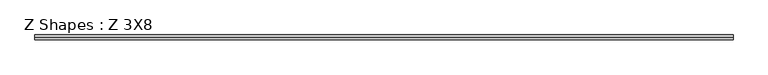
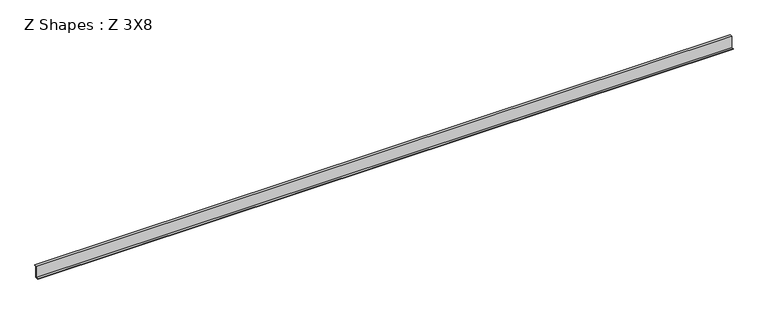
"""IFC4 building model written with IfcOpenShell, lengths in millimetres: beam geometry, Z Shapes : Z 3X8."""

import ifcopenshell
import ifcopenshell.guid

model = None  # the IFC model being written
_history = None  # IfcOwnerHistory: only IFC2X3 demands one
_inside = {}  # id of a spatial element -> (the spatial element, [elements in it])
_under = {}  # id of a project, library or spatial element -> (it, [spatial elements below it])
_declared = {}  # id of a project -> (the project, [libraries it declares])
_typed = {}  # id of a type object -> (the type object, [elements of that type])
_made_of = {}  # id of a material, layer set ... -> (it, [elements and type objects made of it])


def new_model(schema):
    """Start an empty IFC model of exactly this schema.

    Asked for "IFC4X3", IfcOpenShell would pick the latest addendum, in which some entities
    have other attributes; the version numbers below select the first issue.
    IFC2X3 requires an IfcOwnerHistory on every rooted entity: one is made here for all.
    """
    global model, _history
    if schema == "IFC4X3":
        model = ifcopenshell.file(schema_version=(4, 3, 0, 0))
    else:
        model = ifcopenshell.file(schema=schema)
    _inside.clear()
    _under.clear()
    _declared.clear()
    _typed.clear()
    _made_of.clear()
    _history = None
    if model.schema == "IFC2X3":
        org = make("IfcOrganization", Name="unknown")
        user = make(
            "IfcPersonAndOrganization",
            ThePerson=make("IfcPerson", FamilyName="unknown"),
            TheOrganization=org,
        )
        app = make(
            "IfcApplication",
            ApplicationDeveloper=org,
            Version="unknown",
            ApplicationFullName="unknown",
            ApplicationIdentifier="unknown",
        )
        _history = make(
            "IfcOwnerHistory",
            OwningUser=user,
            OwningApplication=app,
            ChangeAction="ADDED",
            CreationDate=0,
        )
    return model


def make(cls, **values):
    """One entity of the class cls with the attributes given. An attribute that is None is left unset."""
    return model.create_entity(
        cls, **{name: value for name, value in values.items() if value is not None}
    )


def rooted(cls, **values):
    """An entity with a GlobalId (a new one), such as an element, a storey or a relation."""
    return make(cls, GlobalId=ifcopenshell.guid.new(), OwnerHistory=_history, **values)


def si_unit(unit_type, name, prefix=None):
    """IfcSIUnit, for example si_unit("LENGTHUNIT", "METRE", prefix="MILLI")."""
    return make("IfcSIUnit", UnitType=unit_type, Prefix=prefix, Name=name)


def assignment(units):
    """IfcUnitAssignment: the units of a project."""
    return None if units is None else make("IfcUnitAssignment", Units=units)


def point(xyz):
    """IfcCartesianPoint."""
    return None if xyz is None else make("IfcCartesianPoint", Coordinates=xyz)


def direction(xyz):
    """IfcDirection."""
    return None if xyz is None else make("IfcDirection", DirectionRatios=xyz)


def frame(location, z_axis=None, x_axis=None):
    """IfcAxis2Placement3D, a coordinate frame: its origin and axes. An axis left out is left unset."""
    return make(
        "IfcAxis2Placement3D",
        Location=point(location),
        Axis=direction(z_axis),
        RefDirection=direction(x_axis),
    )


def origin():
    """The frame at (0, 0, 0) with its axes left unset."""
    return frame((0.0, 0.0, 0.0))


def place(relative_to, where):
    """IfcLocalPlacement: puts the frame where relative to a parent placement (None: the world)."""
    return make(
        "IfcLocalPlacement", PlacementRelTo=relative_to, RelativePlacement=where
    )


def context(
    kind, dimensions, precision=None, world=None, true_north=None, identifier=None
):
    """IfcGeometricRepresentationContext, for example the 3D "Model" context."""
    return make(
        "IfcGeometricRepresentationContext",
        ContextIdentifier=identifier,
        ContextType=kind,
        CoordinateSpaceDimension=dimensions,
        Precision=precision,
        WorldCoordinateSystem=world,
        TrueNorth=true_north,
    )


def project(units=None, contexts=None):
    """IfcProject with its units and contexts."""
    return rooted(
        "IfcProject",
        Name="project",
        RepresentationContexts=contexts,
        UnitsInContext=assignment(units),
    )


def spatial(cls, under=None, at=None, **own):
    """A site, building, storey or space (cls), placed at a placement, below another one or the project."""
    s = rooted(cls, ObjectPlacement=at, **own)
    if under is not None:
        _under.setdefault(under.id(), (under, []))[1].append(s)
    return s


def polyline(points):
    """IfcPolyline through the points."""
    return make("IfcPolyline", Points=[point(p) for p in points])


def outline(outer, holes=None, kind="AREA"):
    """IfcArbitraryClosedProfileDef: a profile drawn as a closed curve; with holes, ...WithVoids."""
    if holes is None:
        return make("IfcArbitraryClosedProfileDef", ProfileType=kind, OuterCurve=outer)
    return make(
        "IfcArbitraryProfileDefWithVoids",
        ProfileType=kind,
        OuterCurve=outer,
        InnerCurves=holes,
    )


def extrude(swept, where, along, depth):
    """IfcExtrudedAreaSolid: the profile swept, set in the frame where, extruded along a direction by depth."""
    return make(
        "IfcExtrudedAreaSolid",
        SweptArea=swept,
        Position=where,
        ExtrudedDirection=direction(along),
        Depth=depth,
    )


def shape(context_of_items, identifier, shape_type, items):
    """IfcShapeRepresentation: the items that make up one representation, for example the "Body"."""
    return make(
        "IfcShapeRepresentation",
        ContextOfItems=context_of_items,
        RepresentationIdentifier=identifier,
        RepresentationType=shape_type,
        Items=items,
    )


def source(mapping_origin, context_of_items, identifier, shape_type, items):
    """IfcRepresentationMap: a shape defined once, which mapped items show again and again."""
    return make(
        "IfcRepresentationMap",
        MappingOrigin=mapping_origin,
        MappedRepresentation=shape(context_of_items, identifier, shape_type, items),
    )


def transform(
    local_origin,
    x_axis=None,
    y_axis=None,
    z_axis=None,
    scale=None,
    scale2=None,
    scale3=None,
    uniform=True,
):
    """IfcCartesianTransformationOperator3D, or its non-uniform kind. x_axis, y_axis, z_axis: its Axis1, 2, 3."""
    if uniform:
        return make(
            "IfcCartesianTransformationOperator3D",
            Axis1=direction(x_axis),
            Axis2=direction(y_axis),
            LocalOrigin=point(local_origin),
            Scale=scale,
            Axis3=direction(z_axis),
        )
    return make(
        "IfcCartesianTransformationOperator3DnonUniform",
        Axis1=direction(x_axis),
        Axis2=direction(y_axis),
        LocalOrigin=point(local_origin),
        Scale=scale,
        Axis3=direction(z_axis),
        Scale2=scale2,
        Scale3=scale3,
    )


def mapped(mapping_source, mapping_target):
    """IfcMappedItem: shows the shape of a source again, moved by a transform."""
    return make(
        "IfcMappedItem", MappingSource=mapping_source, MappingTarget=mapping_target
    )


def made_of(thing, what):
    """Note that an element or type object is made of a material, layer set ...; save() writes the relation."""
    if what is not None:
        _made_of.setdefault(what.id(), (what, []))[1].append(thing)
    return thing


def element(
    cls,
    number,
    at=None,
    inside=None,
    cuts=None,
    type_object=None,
    material=None,
    context=None,
    identifier="Body",
    shape_type=None,
    held_by="IfcProductDefinitionShape",
    body=None,
    shapes=None,
    **own,
):
    """One element of the class cls, such as IfcWall. Its Tag is "e" and its number.

    at: its placement. inside: the storey or other place that contains it. cuts: it is an
    opening in that element (IfcRelVoidsElement). A single representation is given by context,
    identifier, shape_type and body (its items); several are given by shapes. held_by: the class
    of the entity that holds the representations. save() writes the other relations.
    """
    e = rooted(cls, Tag="e%d" % number, ObjectPlacement=at, **own)
    if body is not None:
        shapes = [shape(context, identifier, shape_type, body)]
    if shapes is not None:
        e.Representation = make(held_by, Representations=shapes)
    if inside is not None:
        _inside.setdefault(inside.id(), (inside, []))[1].append(e)
    if cuts is not None:
        rooted(
            "IfcRelVoidsElement", RelatingBuildingElement=cuts, RelatedOpeningElement=e
        )
    if type_object is not None:
        _typed.setdefault(type_object.id(), (type_object, []))[1].append(e)
    return made_of(e, material)


def aggregate(whole, parts):
    """IfcRelAggregates: a whole, such as a stair, and the parts it consists of."""
    return rooted("IfcRelAggregates", RelatingObject=whole, RelatedObjects=parts)


def save(model, path):
    """Write the relations noted so far, then the file.

    IfcRelAggregates (storeys below a building ...), IfcRelContainedInSpatialStructure (elements
    in a storey), IfcRelDefinesByType, IfcRelAssociatesMaterial and IfcRelDeclares: one each for
    every whole, place, type object, material and project.
    """
    for whole, parts in _under.values():
        aggregate(whole, parts)
    for where, things in _inside.values():
        rooted(
            "IfcRelContainedInSpatialStructure",
            RelatedElements=things,
            RelatingStructure=where,
        )
    for kind, things in _typed.values():
        rooted("IfcRelDefinesByType", RelatedObjects=things, RelatingType=kind)
    for what, things in _made_of.values():
        rooted("IfcRelAssociatesMaterial", RelatedObjects=things, RelatingMaterial=what)
    for by, libraries in _declared.values():
        rooted("IfcRelDeclares", RelatingContext=by, RelatedDefinitions=libraries)
    model.write(path)


def z_shapes_z_3x8_9649d549(model_context):
    return source(origin(), model_context, "Body", "SweptSolid", [
        extrude(outline(polyline([(57.2805719, 92.452825), (27.1991352, 92.452825), (27.1991352, -98.809175), (-18.9194281, -98.809175), (-18.9194281, -92.459175), (19.1805719, -92.459175), (19.1805719, 102.104825), (57.2805719, 102.104825), (57.2805719, 92.452825)])), frame((-11474.45, 0.0, 0.0), z_axis=(1.0, 0.0, 0.0), x_axis=(0.0, 1.0, 0.0)), (0.0, 0.0, 1.0), 11315.7),
    ])


if __name__ == "__main__":
    model = new_model("IFC4")
    model_context = context("Model", 3, world=origin())
    ifc_project = project(units=[si_unit("LENGTHUNIT", "METRE", prefix="MILLI")], contexts=[model_context])
    site = spatial("IfcSite", under=ifc_project)
    building = spatial("IfcBuilding", under=site)
    placement = place(None, origin())
    z_shapes_z_3x8_shape = z_shapes_z_3x8_9649d549(model_context)
    element("IfcBeam", 1, ObjectType="Z Shapes : Z 3X8", at=placement, inside=building, context=model_context, shape_type="MappedRepresentation", body=[
        mapped(z_shapes_z_3x8_shape, transform((0.0, 0.0, 0.0), x_axis=(1.0, 0.0, 0.0), y_axis=(0.0, 1.0, 0.0), z_axis=(0.0, 0.0, 1.0))),
    ])
    save(model, "model.ifc")

# Revit data of these elements
# Type "Z Shapes : Z 3X8"
#   Section Name Key = "W12x26"
#   Assembly Code = "B10"
#   Width = 76.2 mm
#   Web Thickness = 5.842 mm
#   Web Fillet = 7.62 mm
#   Warping Constant = 163001.3 cm⁶
#   Torsional Moment of Inertia = 12.4869 cm⁴
#   Section Area = 7.65 in²
#   Plastic Modulus weak axis = 0.00472801 (stored number, unit not read)
#   Plastic Modulus strong axis = 0.0215278 (stored number, unit not read)
#   Perimeter = 15.0571 m²/m
#   Nominal Weight = 379.441 N/m
#   Moment of Inertia weak axis = 720.08 cm⁴
#   Moment of Inertia strong axis = 8491.12 cm⁴
#   Height = 184.912 mm
#   Flange Thickness = 9.652 mm
#   Elastic Modulus weak axis = 0.00309028 (stored number, unit not read)
#   Elastic Modulus strong axis = 0.0193287 (stored number, unit not read)
#   Centroid Vertical = 92.456 mm
#   Centroid Horizontal = 38.1 mm
#   Length [instance default] = 5' - 0"
#   Structural Material [instance default] = Steel ASTM A992
#   Principal Axes Angle = 0
# Element 1 (IfcBeam, "Z Shapes : Z 3X8")
#   Materials on its faces: "Steel ASTM A992"
# Materials
#   "Steel ASTM A992": class "Metal", colour RGB 189 187 185, transparency 0, Description = "Structural steel 50ksi", Cost = 0
